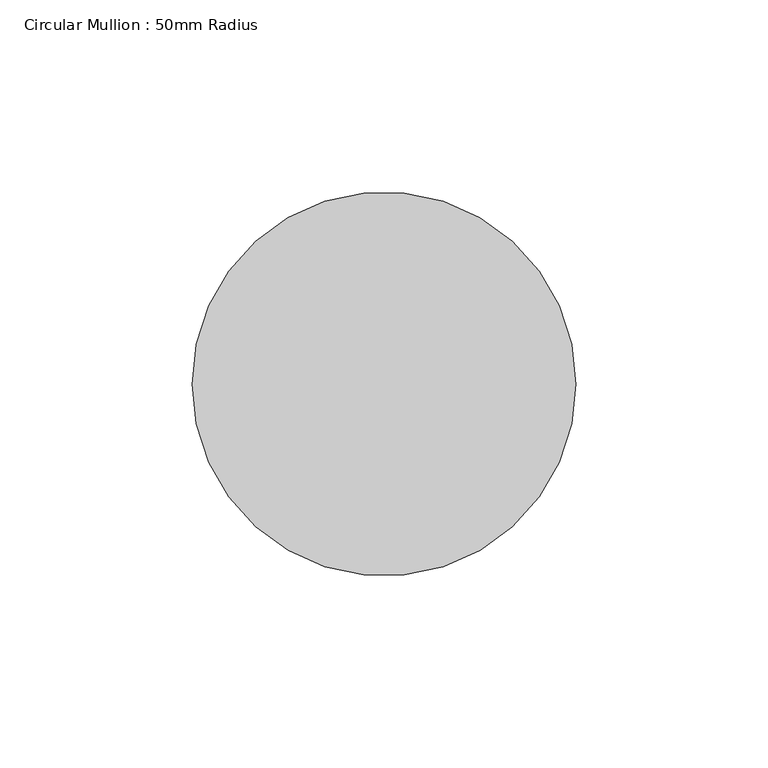
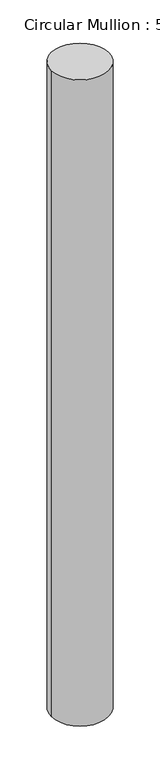
"""IFC4 building model written with IfcOpenShell, lengths in millimetres: member geometry, Circular Mullion : 50mm Radius."""

import ifcopenshell
import ifcopenshell.guid

model = None  # the IFC model being written
_history = None  # IfcOwnerHistory: only IFC2X3 demands one
_inside = {}  # id of a spatial element -> (the spatial element, [elements in it])
_under = {}  # id of a project, library or spatial element -> (it, [spatial elements below it])
_declared = {}  # id of a project -> (the project, [libraries it declares])
_typed = {}  # id of a type object -> (the type object, [elements of that type])
_made_of = {}  # id of a material, layer set ... -> (it, [elements and type objects made of it])


def new_model(schema):
    """Start an empty IFC model of exactly this schema.

    Asked for "IFC4X3", IfcOpenShell would pick the latest addendum, in which some entities
    have other attributes; the version numbers below select the first issue.
    IFC2X3 requires an IfcOwnerHistory on every rooted entity: one is made here for all.
    """
    global model, _history
    if schema == "IFC4X3":
        model = ifcopenshell.file(schema_version=(4, 3, 0, 0))
    else:
        model = ifcopenshell.file(schema=schema)
    _inside.clear()
    _under.clear()
    _declared.clear()
    _typed.clear()
    _made_of.clear()
    _history = None
    if model.schema == "IFC2X3":
        org = make("IfcOrganization", Name="unknown")
        user = make(
            "IfcPersonAndOrganization",
            ThePerson=make("IfcPerson", FamilyName="unknown"),
            TheOrganization=org,
        )
        app = make(
            "IfcApplication",
            ApplicationDeveloper=org,
            Version="unknown",
            ApplicationFullName="unknown",
            ApplicationIdentifier="unknown",
        )
        _history = make(
            "IfcOwnerHistory",
            OwningUser=user,
            OwningApplication=app,
            ChangeAction="ADDED",
            CreationDate=0,
        )
    return model


def make(cls, **values):
    """One entity of the class cls with the attributes given. An attribute that is None is left unset."""
    return model.create_entity(
        cls, **{name: value for name, value in values.items() if value is not None}
    )


def rooted(cls, **values):
    """An entity with a GlobalId (a new one), such as an element, a storey or a relation."""
    return make(cls, GlobalId=ifcopenshell.guid.new(), OwnerHistory=_history, **values)


def si_unit(unit_type, name, prefix=None):
    """IfcSIUnit, for example si_unit("LENGTHUNIT", "METRE", prefix="MILLI")."""
    return make("IfcSIUnit", UnitType=unit_type, Prefix=prefix, Name=name)


def assignment(units):
    """IfcUnitAssignment: the units of a project."""
    return None if units is None else make("IfcUnitAssignment", Units=units)


def point(xyz):
    """IfcCartesianPoint."""
    return None if xyz is None else make("IfcCartesianPoint", Coordinates=xyz)


def direction(xyz):
    """IfcDirection."""
    return None if xyz is None else make("IfcDirection", DirectionRatios=xyz)


def frame(location, z_axis=None, x_axis=None):
    """IfcAxis2Placement3D, a coordinate frame: its origin and axes. An axis left out is left unset."""
    return make(
        "IfcAxis2Placement3D",
        Location=point(location),
        Axis=direction(z_axis),
        RefDirection=direction(x_axis),
    )


def origin():
    """The frame at (0, 0, 0) with its axes left unset."""
    return frame((0.0, 0.0, 0.0))


def place(relative_to, where):
    """IfcLocalPlacement: puts the frame where relative to a parent placement (None: the world)."""
    return make(
        "IfcLocalPlacement", PlacementRelTo=relative_to, RelativePlacement=where
    )


def context(
    kind, dimensions, precision=None, world=None, true_north=None, identifier=None
):
    """IfcGeometricRepresentationContext, for example the 3D "Model" context."""
    return make(
        "IfcGeometricRepresentationContext",
        ContextIdentifier=identifier,
        ContextType=kind,
        CoordinateSpaceDimension=dimensions,
        Precision=precision,
        WorldCoordinateSystem=world,
        TrueNorth=true_north,
    )


def project(units=None, contexts=None):
    """IfcProject with its units and contexts."""
    return rooted(
        "IfcProject",
        Name="project",
        RepresentationContexts=contexts,
        UnitsInContext=assignment(units),
    )


def spatial(cls, under=None, at=None, **own):
    """A site, building, storey or space (cls), placed at a placement, below another one or the project."""
    s = rooted(cls, ObjectPlacement=at, **own)
    if under is not None:
        _under.setdefault(under.id(), (under, []))[1].append(s)
    return s


def ellipse_curve(where, semi_axis1, semi_axis2):
    """IfcEllipse in the frame where."""
    return make(
        "IfcEllipse", Position=where, SemiAxis1=semi_axis1, SemiAxis2=semi_axis2
    )


def shape(context_of_items, identifier, shape_type, items):
    """IfcShapeRepresentation: the items that make up one representation, for example the "Body"."""
    return make(
        "IfcShapeRepresentation",
        ContextOfItems=context_of_items,
        RepresentationIdentifier=identifier,
        RepresentationType=shape_type,
        Items=items,
    )


def source(mapping_origin, context_of_items, identifier, shape_type, items):
    """IfcRepresentationMap: a shape defined once, which mapped items show again and again."""
    return make(
        "IfcRepresentationMap",
        MappingOrigin=mapping_origin,
        MappedRepresentation=shape(context_of_items, identifier, shape_type, items),
    )


def transform(
    local_origin,
    x_axis=None,
    y_axis=None,
    z_axis=None,
    scale=None,
    scale2=None,
    scale3=None,
    uniform=True,
):
    """IfcCartesianTransformationOperator3D, or its non-uniform kind. x_axis, y_axis, z_axis: its Axis1, 2, 3."""
    if uniform:
        return make(
            "IfcCartesianTransformationOperator3D",
            Axis1=direction(x_axis),
            Axis2=direction(y_axis),
            LocalOrigin=point(local_origin),
            Scale=scale,
            Axis3=direction(z_axis),
        )
    return make(
        "IfcCartesianTransformationOperator3DnonUniform",
        Axis1=direction(x_axis),
        Axis2=direction(y_axis),
        LocalOrigin=point(local_origin),
        Scale=scale,
        Axis3=direction(z_axis),
        Scale2=scale2,
        Scale3=scale3,
    )


def mapped(mapping_source, mapping_target):
    """IfcMappedItem: shows the shape of a source again, moved by a transform."""
    return make(
        "IfcMappedItem", MappingSource=mapping_source, MappingTarget=mapping_target
    )


def made_of(thing, what):
    """Note that an element or type object is made of a material, layer set ...; save() writes the relation."""
    if what is not None:
        _made_of.setdefault(what.id(), (what, []))[1].append(thing)
    return thing


def element(
    cls,
    number,
    at=None,
    inside=None,
    cuts=None,
    type_object=None,
    material=None,
    context=None,
    identifier="Body",
    shape_type=None,
    held_by="IfcProductDefinitionShape",
    body=None,
    shapes=None,
    **own,
):
    """One element of the class cls, such as IfcWall. Its Tag is "e" and its number.

    at: its placement. inside: the storey or other place that contains it. cuts: it is an
    opening in that element (IfcRelVoidsElement). A single representation is given by context,
    identifier, shape_type and body (its items); several are given by shapes. held_by: the class
    of the entity that holds the representations. save() writes the other relations.
    """
    e = rooted(cls, Tag="e%d" % number, ObjectPlacement=at, **own)
    if body is not None:
        shapes = [shape(context, identifier, shape_type, body)]
    if shapes is not None:
        e.Representation = make(held_by, Representations=shapes)
    if inside is not None:
        _inside.setdefault(inside.id(), (inside, []))[1].append(e)
    if cuts is not None:
        rooted(
            "IfcRelVoidsElement", RelatingBuildingElement=cuts, RelatedOpeningElement=e
        )
    if type_object is not None:
        _typed.setdefault(type_object.id(), (type_object, []))[1].append(e)
    return made_of(e, material)


def aggregate(whole, parts):
    """IfcRelAggregates: a whole, such as a stair, and the parts it consists of."""
    return rooted("IfcRelAggregates", RelatingObject=whole, RelatedObjects=parts)


def save(model, path):
    """Write the relations noted so far, then the file.

    IfcRelAggregates (storeys below a building ...), IfcRelContainedInSpatialStructure (elements
    in a storey), IfcRelDefinesByType, IfcRelAssociatesMaterial and IfcRelDeclares: one each for
    every whole, place, type object, material and project.
    """
    for whole, parts in _under.values():
        aggregate(whole, parts)
    for where, things in _inside.values():
        rooted(
            "IfcRelContainedInSpatialStructure",
            RelatedElements=things,
            RelatingStructure=where,
        )
    for kind, things in _typed.values():
        rooted("IfcRelDefinesByType", RelatedObjects=things, RelatingType=kind)
    for what, things in _made_of.values():
        rooted("IfcRelAssociatesMaterial", RelatedObjects=things, RelatingMaterial=what)
    for by, libraries in _declared.values():
        rooted("IfcRelDeclares", RelatingContext=by, RelatedDefinitions=libraries)
    model.write(path)


def plane_surface(at):
    """IfcPlane: the flat surface through the origin of the frame at, square to its z axis."""
    return make("IfcPlane", Position=at)


def cylinder_surface(at, radius):
    """IfcCylindricalSurface: all points at the distance radius from the z axis of the frame at."""
    return make("IfcCylindricalSurface", Position=at, Radius=radius)


def advanced_brep(points, edges, surfaces, faces):
    """IfcAdvancedBrep: a solid bounded by faces that lie on surfaces and meet in shared edges.

    An edge is (start, end): straight between two places in points (the first is 0);
    or (start, end, curve); or (start, end, curve, False) where it runs against its curve.
    A face is (place in surfaces, loops), or (place, loops, False) where it looks against
    its surface's normal. A loop lists edges by number (the first is 1), with a minus sign
    where the edge is run from its end to its start. The first loop is the outer one.
    """
    corners = [point(p) for p in points]
    vertices = [make("IfcVertexPoint", VertexGeometry=c) for c in corners]
    made = []
    for start, end, *more in edges:
        made.append(
            make(
                "IfcEdgeCurve",
                EdgeStart=vertices[start],
                EdgeEnd=vertices[end],
                EdgeGeometry=more[0] if more else make("IfcPolyline", Points=[corners[start], corners[end]]),
                SameSense=more[1] if len(more) > 1 else True,
            )
        )
    hull = []
    for where, loops, *sense in faces:
        bounds = []
        for j, loop in enumerate(loops):
            ring = [make("IfcOrientedEdge", EdgeElement=made[abs(k) - 1], Orientation=k > 0) for k in loop]
            bounds.append(
                make(
                    "IfcFaceOuterBound" if j == 0 else "IfcFaceBound",
                    Bound=make("IfcEdgeLoop", EdgeList=ring),
                    Orientation=True,
                )
            )
        hull.append(make("IfcAdvancedFace", Bounds=bounds, FaceSurface=surfaces[where], SameSense=sense[0] if sense else True))
    return make("IfcAdvancedBrep", Outer=make("IfcClosedShell", CfsFaces=hull))


def circular_mullion_50mm_radius_1c4f4fd8(model_context):
    return source(origin(), model_context, "Body", "AdvancedBrep", [
        advanced_brep(
        [(-100.0, 0.0, 1.324491), (0.0, 0.0, 0.0), (0.0, 0.0, -1185.9270552), (-100.0, 0.0, -1187.1782821)],
        [
            (0, 1, ellipse_curve(frame((-50.0, 0.0, 0.6622455), z_axis=(-0.01324113131648021, -0.019880271076322148, -0.9997146829287803), x_axis=(-0.5541830862624147, -0.8320520140977105, 0.023886245762118827)), 50.0142699, 50.0)),
            (1, 2),
            (2, 3, ellipse_curve(frame((-50.0, 0.0, -1186.5526686), z_axis=(-0.012509082807271947, -0.018781171425677486, 0.9997453628035493), x_axis=(0.5542000933825312, 0.8320775486347379, 0.022565671999725753)), 50.0127351, 50.0)),
            (3, 0),
            (1, 0, ellipse_curve(frame((-50.0, 0.0, 0.6622455), z_axis=(-0.01324113131648021, -0.019880271076322148, -0.9997146829287803), x_axis=(-0.5541830862624147, -0.8320520140977105, 0.023886245762118827)), 50.0142699, 50.0)),
            (3, 2, ellipse_curve(frame((-50.0, 0.0, -1186.5526686), z_axis=(-0.012509082807271947, -0.018781171425677486, 0.9997453628035493), x_axis=(0.5542000933825312, 0.8320775486347379, 0.022565671999725753)), 50.0127351, 50.0)),
        ],
        [
            cylinder_surface(frame((-50.0, 0.0, 0.0), z_axis=(0.0, 0.0, 1.0), x_axis=(1.0, 0.0, 0.0)), 50.0),
            plane_surface(frame((-253.6818337, 168.9632128, 0.0), z_axis=(0.01324113131648021, 0.019880271076322148, 0.9997146829287803), x_axis=(0.5541830862624152, 0.8320520140977102, -0.023886245762118497))),
            plane_surface(frame((-253.6818337, 168.9632128, -1185.9270552), z_axis=(0.012509082807271947, 0.018781171425677486, -0.9997453628035493), x_axis=(0.554200093382531, 0.8320775486347376, 0.022565671999740466))),
        ],
        [
            (0, [[1, 2, 3, 4]]),
            (0, [[5, -4, 6, -2]]),
            (1, [[-1, -5]]),
            (2, [[-6, -3]]),
        ],
    ),
    ])


if __name__ == "__main__":
    model = new_model("IFC4")
    model_context = context("Model", 3, world=origin())
    ifc_project = project(units=[si_unit("LENGTHUNIT", "METRE", prefix="MILLI")], contexts=[model_context])
    site = spatial("IfcSite", under=ifc_project)
    building = spatial("IfcBuilding", under=site)
    placement = place(None, origin())
    circular_mullion_50mm_radius_shape = circular_mullion_50mm_radius_1c4f4fd8(model_context)
    element("IfcMember", 1, ObjectType="Circular Mullion : 50mm Radius", at=placement, inside=building, context=model_context, shape_type="MappedRepresentation", body=[
        mapped(circular_mullion_50mm_radius_shape, transform((0.0, 0.0, 0.0), x_axis=(1.0, 0.0, 0.0), y_axis=(0.0, 1.0, 0.0), z_axis=(0.0, 0.0, 1.0))),
    ])
    save(model, "model.ifc")

# Revit data of these elements
# Type "Circular Mullion : 50mm Radius"
#   built-in parameter 1007350 = 0.164042 (stored number, unit not read)
# Element 1 (IfcMember, "Circular Mullion : 50mm Radius")
#   Materials on its faces: "Aluminium"
# Materials
#   "Aluminium": class "Metal", colour RGB 247 247 247, transparency 0, Description = "Aluminium 6061", Cost = 0
